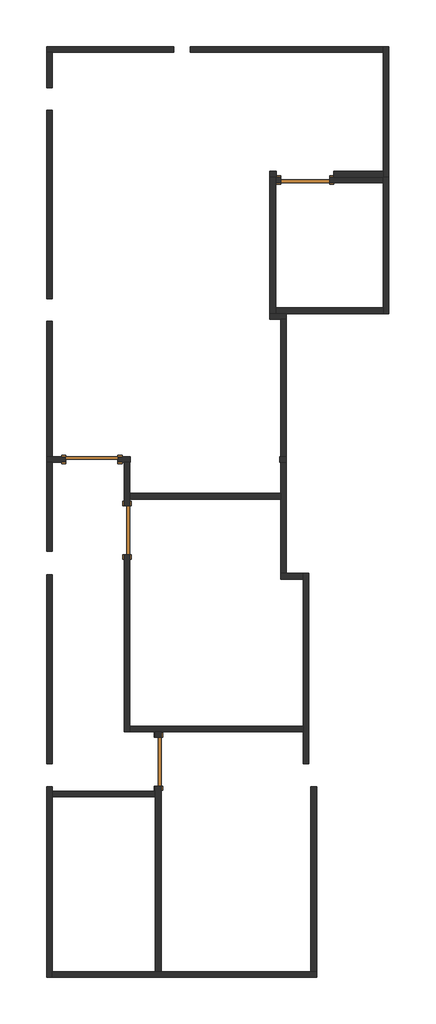
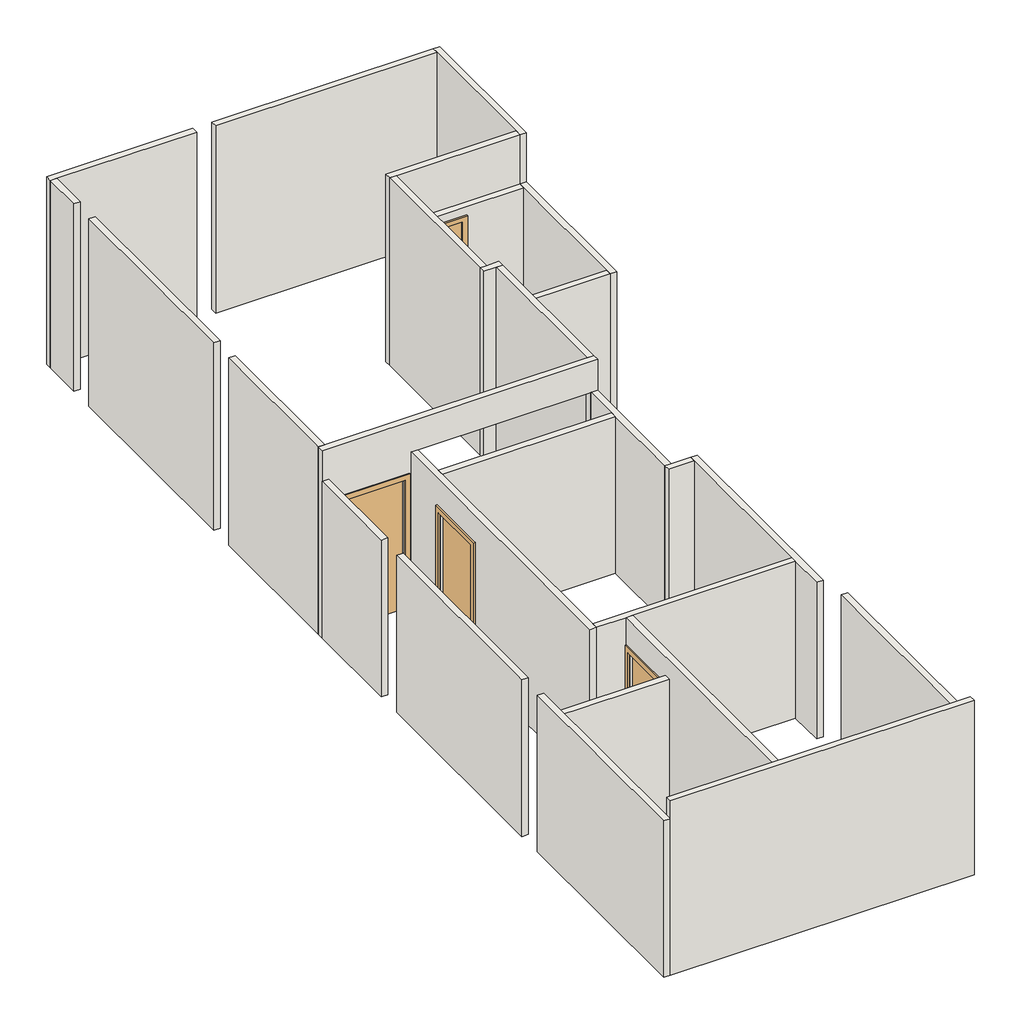
# One storey: 27 walls, 4 doors.
"""IFC4 building model written with IfcOpenShell, lengths in millimetres."""

import ifcopenshell
import ifcopenshell.guid

model = None  # the IFC model being written
_history = None  # IfcOwnerHistory: only IFC2X3 demands one
_inside = {}  # id of a spatial element -> (the spatial element, [elements in it])
_under = {}  # id of a project, library or spatial element -> (it, [spatial elements below it])
_declared = {}  # id of a project -> (the project, [libraries it declares])
_typed = {}  # id of a type object -> (the type object, [elements of that type])
_made_of = {}  # id of a material, layer set ... -> (it, [elements and type objects made of it])


def new_model(schema):
    """Start an empty IFC model of exactly this schema.

    Asked for "IFC4X3", IfcOpenShell would pick the latest addendum, in which some entities
    have other attributes; the version numbers below select the first issue.
    IFC2X3 requires an IfcOwnerHistory on every rooted entity: one is made here for all.
    """
    global model, _history
    if schema == "IFC4X3":
        model = ifcopenshell.file(schema_version=(4, 3, 0, 0))
    else:
        model = ifcopenshell.file(schema=schema)
    _inside.clear()
    _under.clear()
    _declared.clear()
    _typed.clear()
    _made_of.clear()
    _history = None
    if model.schema == "IFC2X3":
        org = make("IfcOrganization", Name="unknown")
        user = make(
            "IfcPersonAndOrganization",
            ThePerson=make("IfcPerson", FamilyName="unknown"),
            TheOrganization=org,
        )
        app = make(
            "IfcApplication",
            ApplicationDeveloper=org,
            Version="unknown",
            ApplicationFullName="unknown",
            ApplicationIdentifier="unknown",
        )
        _history = make(
            "IfcOwnerHistory",
            OwningUser=user,
            OwningApplication=app,
            ChangeAction="ADDED",
            CreationDate=0,
        )
    return model


def make(cls, **values):
    """One entity of the class cls with the attributes given. An attribute that is None is left unset."""
    return model.create_entity(
        cls, **{name: value for name, value in values.items() if value is not None}
    )


def rooted(cls, **values):
    """An entity with a GlobalId (a new one), such as an element, a storey or a relation."""
    return make(cls, GlobalId=ifcopenshell.guid.new(), OwnerHistory=_history, **values)


def si_unit(unit_type, name, prefix=None):
    """IfcSIUnit, for example si_unit("LENGTHUNIT", "METRE", prefix="MILLI")."""
    return make("IfcSIUnit", UnitType=unit_type, Prefix=prefix, Name=name)


def assignment(units):
    """IfcUnitAssignment: the units of a project."""
    return None if units is None else make("IfcUnitAssignment", Units=units)


def point(xyz):
    """IfcCartesianPoint."""
    return None if xyz is None else make("IfcCartesianPoint", Coordinates=xyz)


def direction(xyz):
    """IfcDirection."""
    return None if xyz is None else make("IfcDirection", DirectionRatios=xyz)


def frame(location, z_axis=None, x_axis=None):
    """IfcAxis2Placement3D, a coordinate frame: its origin and axes. An axis left out is left unset."""
    return make(
        "IfcAxis2Placement3D",
        Location=point(location),
        Axis=direction(z_axis),
        RefDirection=direction(x_axis),
    )


def origin():
    """The frame at (0, 0, 0) with its axes left unset."""
    return frame((0.0, 0.0, 0.0))


def origin_with_axes():
    """The frame at (0, 0, 0) with the z axis (0, 0, 1) and the x axis (1, 0, 0) written out."""
    return frame((0.0, 0.0, 0.0), z_axis=(0.0, 0.0, 1.0), x_axis=(1.0, 0.0, 0.0))


def place(relative_to, where):
    """IfcLocalPlacement: puts the frame where relative to a parent placement (None: the world)."""
    return make(
        "IfcLocalPlacement", PlacementRelTo=relative_to, RelativePlacement=where
    )


def context(
    kind, dimensions, precision=None, world=None, true_north=None, identifier=None
):
    """IfcGeometricRepresentationContext, for example the 3D "Model" context."""
    return make(
        "IfcGeometricRepresentationContext",
        ContextIdentifier=identifier,
        ContextType=kind,
        CoordinateSpaceDimension=dimensions,
        Precision=precision,
        WorldCoordinateSystem=world,
        TrueNorth=true_north,
    )


def project(units=None, contexts=None):
    """IfcProject with its units and contexts."""
    return rooted(
        "IfcProject",
        Name="project",
        RepresentationContexts=contexts,
        UnitsInContext=assignment(units),
    )


def spatial(cls, under=None, at=None, **own):
    """A site, building, storey or space (cls), placed at a placement, below another one or the project."""
    s = rooted(cls, ObjectPlacement=at, **own)
    if under is not None:
        _under.setdefault(under.id(), (under, []))[1].append(s)
    return s


def polyline(points):
    """IfcPolyline through the points."""
    return make("IfcPolyline", Points=[point(p) for p in points])


def outline(outer, holes=None, kind="AREA"):
    """IfcArbitraryClosedProfileDef: a profile drawn as a closed curve; with holes, ...WithVoids."""
    if holes is None:
        return make("IfcArbitraryClosedProfileDef", ProfileType=kind, OuterCurve=outer)
    return make(
        "IfcArbitraryProfileDefWithVoids",
        ProfileType=kind,
        OuterCurve=outer,
        InnerCurves=holes,
    )


def extrude(swept, where, along, depth):
    """IfcExtrudedAreaSolid: the profile swept, set in the frame where, extruded along a direction by depth."""
    return make(
        "IfcExtrudedAreaSolid",
        SweptArea=swept,
        Position=where,
        ExtrudedDirection=direction(along),
        Depth=depth,
    )


def faces_of(points, faces, orient=None, outer=None):
    """IfcFace entities. A face is a list of loops; a loop is a list of indices into points, from 0.

    orient and outer hold one flag for each loop. By default every Orientation is true, the
    first loop of a face is its IfcFaceOuterBound and the others are IfcFaceBound.
    """
    made = []
    for i, loops in enumerate(faces):
        bounds = []
        for j, loop in enumerate(loops):
            is_outer = j == 0 if outer is None else outer[i][j]
            bounds.append(
                make(
                    "IfcFaceOuterBound" if is_outer else "IfcFaceBound",
                    Bound=make("IfcPolyLoop", Polygon=[points[k] for k in loop]),
                    Orientation=True if orient is None else orient[i][j],
                )
            )
        made.append(make("IfcFace", Bounds=bounds))
    return made


def faceted_brep(points, faces, orient=None, outer=None, voids=None):
    """IfcFacetedBrep: a solid bounded by flat faces; with voids (closed shells), ...WithVoids."""
    shared = [point(p) for p in points]
    hull = make("IfcClosedShell", CfsFaces=faces_of(shared, faces, orient, outer))
    if voids is None:
        return make("IfcFacetedBrep", Outer=hull)
    return make(
        "IfcFacetedBrepWithVoids",
        Outer=hull,
        Voids=[
            make(cls, CfsFaces=faces_of(shared, fs, o, b)) for cls, fs, o, b in voids
        ],
    )


def shape(context_of_items, identifier, shape_type, items):
    """IfcShapeRepresentation: the items that make up one representation, for example the "Body"."""
    return make(
        "IfcShapeRepresentation",
        ContextOfItems=context_of_items,
        RepresentationIdentifier=identifier,
        RepresentationType=shape_type,
        Items=items,
    )


def source(mapping_origin, context_of_items, identifier, shape_type, items):
    """IfcRepresentationMap: a shape defined once, which mapped items show again and again."""
    return make(
        "IfcRepresentationMap",
        MappingOrigin=mapping_origin,
        MappedRepresentation=shape(context_of_items, identifier, shape_type, items),
    )


def transform(
    local_origin,
    x_axis=None,
    y_axis=None,
    z_axis=None,
    scale=None,
    scale2=None,
    scale3=None,
    uniform=True,
):
    """IfcCartesianTransformationOperator3D, or its non-uniform kind. x_axis, y_axis, z_axis: its Axis1, 2, 3."""
    if uniform:
        return make(
            "IfcCartesianTransformationOperator3D",
            Axis1=direction(x_axis),
            Axis2=direction(y_axis),
            LocalOrigin=point(local_origin),
            Scale=scale,
            Axis3=direction(z_axis),
        )
    return make(
        "IfcCartesianTransformationOperator3DnonUniform",
        Axis1=direction(x_axis),
        Axis2=direction(y_axis),
        LocalOrigin=point(local_origin),
        Scale=scale,
        Axis3=direction(z_axis),
        Scale2=scale2,
        Scale3=scale3,
    )


def mapped(mapping_source, mapping_target):
    """IfcMappedItem: shows the shape of a source again, moved by a transform."""
    return make(
        "IfcMappedItem", MappingSource=mapping_source, MappingTarget=mapping_target
    )


def made_of(thing, what):
    """Note that an element or type object is made of a material, layer set ...; save() writes the relation."""
    if what is not None:
        _made_of.setdefault(what.id(), (what, []))[1].append(thing)
    return thing


def element(
    cls,
    number,
    at=None,
    inside=None,
    cuts=None,
    type_object=None,
    material=None,
    context=None,
    identifier="Body",
    shape_type=None,
    held_by="IfcProductDefinitionShape",
    body=None,
    shapes=None,
    **own,
):
    """One element of the class cls, such as IfcWall. Its Tag is "e" and its number.

    at: its placement. inside: the storey or other place that contains it. cuts: it is an
    opening in that element (IfcRelVoidsElement). A single representation is given by context,
    identifier, shape_type and body (its items); several are given by shapes. held_by: the class
    of the entity that holds the representations. save() writes the other relations.
    """
    e = rooted(cls, Tag="e%d" % number, ObjectPlacement=at, **own)
    if body is not None:
        shapes = [shape(context, identifier, shape_type, body)]
    if shapes is not None:
        e.Representation = make(held_by, Representations=shapes)
    if inside is not None:
        _inside.setdefault(inside.id(), (inside, []))[1].append(e)
    if cuts is not None:
        rooted(
            "IfcRelVoidsElement", RelatingBuildingElement=cuts, RelatedOpeningElement=e
        )
    if type_object is not None:
        _typed.setdefault(type_object.id(), (type_object, []))[1].append(e)
    return made_of(e, material)


def aggregate(whole, parts):
    """IfcRelAggregates: a whole, such as a stair, and the parts it consists of."""
    return rooted("IfcRelAggregates", RelatingObject=whole, RelatedObjects=parts)


def save(model, path):
    """Write the relations noted so far, then the file.

    IfcRelAggregates (storeys below a building ...), IfcRelContainedInSpatialStructure (elements
    in a storey), IfcRelDefinesByType, IfcRelAssociatesMaterial and IfcRelDeclares: one each for
    every whole, place, type object, material and project.
    """
    for whole, parts in _under.values():
        aggregate(whole, parts)
    for where, things in _inside.values():
        rooted(
            "IfcRelContainedInSpatialStructure",
            RelatedElements=things,
            RelatingStructure=where,
        )
    for kind, things in _typed.values():
        rooted("IfcRelDefinesByType", RelatedObjects=things, RelatingType=kind)
    for what, things in _made_of.values():
        rooted("IfcRelAssociatesMaterial", RelatedObjects=things, RelatingMaterial=what)
    for by, libraries in _declared.values():
        rooted("IfcRelDeclares", RelatingContext=by, RelatedDefinitions=libraries)
    model.write(path)


def m_single_flush_0864_x_2032mm_0d7903e5(model_context):
    return source(origin(), model_context, "Body", "SweptSolid", [
        extrude(outline(polyline([(2108.0, -508.0), (0.0, -508.0), (0.0, -432.0), (2032.0, -432.0), (2032.0, 432.0), (0.0, 432.0), (0.0, 508.0), (2108.0, 508.0), (2108.0, -508.0)])), frame((0.0, -75.0, 0.0), z_axis=(0.0, 1.0, 0.0), x_axis=(0.0, 0.0, 1.0)), (0.0, 0.0, 1.0), 25.0),
        extrude(outline(polyline([(2108.0, 508.0), (2108.0, -508.0), (0.0, -508.0), (0.0, -432.0), (2032.0, -432.0), (2032.0, 432.0), (0.0, 432.0), (0.0, 508.0), (2108.0, 508.0)])), frame((0.0, 50.0, 0.0), z_axis=(0.0, 1.0, 0.0), x_axis=(0.0, 0.0, 1.0)), (0.0, 0.0, 1.0), 25.0),
        extrude(outline(polyline([(432.0, 1.0), (432.0, -50.0), (-432.0, -50.0), (-432.0, 1.0), (432.0, 1.0)])), origin_with_axes(), (0.0, 0.0, 1.0), 2032.0),
    ])


def m_single_flush_0864_x_2032mm_252f296b(model_context):
    return source(origin(), model_context, "Body", "SweptSolid", [
        extrude(outline(polyline([(2108.0, -508.0), (0.0, -508.0), (0.0, -432.0), (2032.0, -432.0), (2032.0, 432.0), (0.0, 432.0), (0.0, 508.0), (2108.0, 508.0), (2108.0, -508.0)])), frame((0.0, 50.0, 0.0), z_axis=(0.0, 1.0, 0.0), x_axis=(0.0, 0.0, 1.0)), (0.0, 0.0, 1.0), 25.0),
        extrude(outline(polyline([(2108.0, 508.0), (2108.0, -508.0), (0.0, -508.0), (0.0, -432.0), (2032.0, -432.0), (2032.0, 432.0), (0.0, 432.0), (0.0, 508.0), (2108.0, 508.0)])), frame((0.0, -75.0, 0.0), z_axis=(0.0, 1.0, 0.0), x_axis=(0.0, 0.0, 1.0)), (0.0, 0.0, 1.0), 25.0),
        extrude(outline(polyline([(432.0, -1.0), (-432.0, -1.0), (-432.0, 50.0), (432.0, 50.0), (432.0, -1.0)])), origin_with_axes(), (0.0, 0.0, 1.0), 2032.0),
    ])


def m_single_flush_0915_x_2134mm_17617764(model_context):
    return source(origin(), model_context, "Body", "SweptSolid", [
        extrude(outline(polyline([(2210.0, -533.5), (0.0, -533.5), (0.0, -457.5), (2134.0, -457.5), (2134.0, 457.5), (0.0, 457.5), (0.0, 533.5), (2210.0, 533.5), (2210.0, -533.5)])), frame((0.0, -75.0, 0.0), z_axis=(0.0, 1.0, 0.0), x_axis=(0.0, 0.0, 1.0)), (0.0, 0.0, 1.0), 25.0),
        extrude(outline(polyline([(2210.0, 533.5), (2210.0, -533.5), (0.0, -533.5), (0.0, -457.5), (2134.0, -457.5), (2134.0, 457.5), (0.0, 457.5), (0.0, 533.5), (2210.0, 533.5)])), frame((0.0, 50.0, 0.0), z_axis=(0.0, 1.0, 0.0), x_axis=(0.0, 0.0, 1.0)), (0.0, 0.0, 1.0), 25.0),
        extrude(outline(polyline([(457.5, 1.0), (457.5, -50.0), (-457.5, -50.0), (-457.5, 1.0), (457.5, 1.0)])), origin_with_axes(), (0.0, 0.0, 1.0), 2134.0),
    ])


model = new_model("IFC4")

# Units and contexts
model_context = context("Model", 3, world=origin())
ifc_project = project(units=[si_unit("LENGTHUNIT", "METRE", prefix="MILLI")], contexts=[model_context])

# Site, building, storey
site = spatial("IfcSite", under=ifc_project)
building = spatial("IfcBuilding", under=site)
storey = spatial("IfcBuildingStorey", under=building, Name="Suelo de apartemento", Elevation=250.0)

# Doors
placement = place(None, origin())
m_single_flush_0864_x_2032mm_shape = m_single_flush_0864_x_2032mm_0d7903e5(model_context)
element("IfcDoor", 1, ObjectType="M_Single-Flush : 0864 x 2032mm", at=placement, inside=storey, context=model_context, shape_type="MappedRepresentation", body=[
    mapped(m_single_flush_0864_x_2032mm_shape, transform((7037.3508412, 6265.939444, 250.0), x_axis=(0.0, 1.0, 0.0), y_axis=(-1.0, 0.0, 0.0), z_axis=(0.0, 0.0, 1.0))),
])
element("IfcDoor", 2, ObjectType="M_Single-Flush : 0864 x 2032mm", at=placement, inside=storey, context=model_context, shape_type="MappedRepresentation", body=[
    mapped(m_single_flush_0864_x_2032mm_shape, transform((7592.3508412, 2190.939444, 250.0), x_axis=(0.0, 1.0, 0.0), y_axis=(-1.0, 0.0, 0.0), z_axis=(0.0, 0.0, 1.0))),
])
m_single_flush_0864_x_2032mm_2_shape = m_single_flush_0864_x_2032mm_252f296b(model_context)
element("IfcDoor", 3, ObjectType="M_Single-Flush : 0864 x 2032mm", at=placement, inside=storey, context=model_context, shape_type="MappedRepresentation", body=[
    mapped(m_single_flush_0864_x_2032mm_2_shape, transform((10177.3508412, 12440.939444, 250.0), x_axis=(-1.0, 0.0, 0.0), y_axis=(0.0, -1.0, 0.0), z_axis=(0.0, 0.0, 1.0))),
])
m_single_flush_0915_x_2134mm_shape = m_single_flush_0915_x_2134mm_17617764(model_context)
element("IfcDoor", 4, ObjectType="M_Single-Flush : 0915 x 2134mm", at=placement, inside=storey, context=model_context, shape_type="MappedRepresentation", body=[
    mapped(m_single_flush_0915_x_2134mm_shape, transform((6422.3508412, 7515.939444, 250.0), x_axis=(-1.0, 0.0, 0.0), y_axis=(0.0, -1.0, 0.0), z_axis=(0.0, 0.0, 1.0))),
])

# Walls
element("IfcWall", 5, ObjectType="Steel Frame 100mm", at=placement, inside=storey, context=model_context, shape_type="Brep", body=[
    faceted_brep([(5722.3508412, -1614.060556, 250.0), (5722.3508412, -1514.060556, 250.0), (5722.3508412, 1565.939444, 250.0), (5722.3508412, 1665.939444, 250.0), (5722.3508412, 1745.939444, 250.0), (5722.3508412, 1745.939444, 2790.0), (5722.3508412, -1614.060556, 2790.0), (5622.3508412, -1614.060556, 250.0), (5622.3508412, -1614.060556, 2790.0), (5622.3508412, 1745.939444, 2790.0), (5622.3508412, 1745.939444, 250.0)], [[[0, 1, 2, 3, 4, 5, 6]], [[7, 8, 9, 10]], [[4, 3, 2, 1, 0, 7, 10]], [[5, 4, 10, 9]], [[6, 5, 9, 8]], [[0, 6, 8, 7]]]),
])
element("IfcWall", 6, ObjectType="Steel Frame 100mm", at=placement, inside=storey, context=model_context, shape_type="SweptSolid", body=[
    extrude(outline(polyline([(5722.3508412, 5485.939444), (5722.3508412, 2155.939444), (5622.3508412, 2155.939444), (5622.3508412, 5485.939444), (5722.3508412, 5485.939444)])), frame((0.0, 0.0, 250.0), z_axis=(0.0, 0.0, 1.0), x_axis=(1.0, 0.0, 0.0)), (0.0, 0.0, 1.0), 2540.0),
])
element("IfcWall", 7, ObjectType="Steel Frame 100mm", at=placement, inside=storey, context=model_context, shape_type="SweptSolid", body=[
    extrude(outline(polyline([(5722.3508412, 9945.939444), (5722.3508412, 7565.939444), (5622.3508412, 7565.939444), (5622.3508412, 9945.939444), (5722.3508412, 9945.939444)])), frame((0.0, 0.0, 250.0), z_axis=(0.0, 0.0, 1.0), x_axis=(1.0, 0.0, 0.0)), (0.0, 0.0, 1.0), 3040.0),
])
element("IfcWall", 8, ObjectType="Steel Frame 100mm", at=placement, inside=storey, context=model_context, shape_type="SweptSolid", body=[
    extrude(outline(polyline([(5722.3508412, 13665.939444), (5722.3508412, 10345.939444), (5622.3508412, 10345.939444), (5622.3508412, 13665.939444), (5722.3508412, 13665.939444)])), frame((0.0, 0.0, 250.0), z_axis=(0.0, 0.0, 1.0), x_axis=(1.0, 0.0, 0.0)), (0.0, 0.0, 1.0), 3040.0),
])
element("IfcWall", 9, ObjectType="Steel Frame 100mm", at=placement, inside=storey, context=model_context, shape_type="SweptSolid", body=[
    extrude(outline(polyline([(5722.3508412, 14690.939444), (5722.3508412, 14065.939444), (5622.3508412, 14065.939444), (5622.3508412, 14690.939444), (5722.3508412, 14690.939444)])), frame((0.0, 0.0, 250.0), z_axis=(0.0, 0.0, 1.0), x_axis=(1.0, 0.0, 0.0)), (0.0, 0.0, 1.0), 3040.0),
])
element("IfcWall", 10, ObjectType="Steel Frame 100mm", at=placement, inside=storey, context=model_context, shape_type="Brep", body=[
    faceted_brep([(5622.3508412, 14690.939444, 250.0), (5722.3508412, 14690.939444, 250.0), (7867.3508412, 14690.939444, 250.0), (7867.3508412, 14690.939444, 3290.0), (5722.3508412, 14690.939444, 3290.0), (5622.3508412, 14690.939444, 3290.0), (5622.3508412, 14790.939444, 250.0), (5622.3508412, 14790.939444, 3290.0), (7867.3508412, 14790.939444, 3290.0), (7867.3508412, 14790.939444, 250.0)], [[[0, 1, 2, 3, 4, 5]], [[6, 7, 8, 9]], [[2, 1, 0, 6, 9]], [[3, 2, 9, 8]], [[5, 4, 3, 8, 7]], [[0, 5, 7, 6]]]),
])
element("IfcWall", 11, ObjectType="Steel Frame 100mm", at=placement, inside=storey, context=model_context, shape_type="Brep", body=[
    faceted_brep([(11657.3508412, 12490.939444, 3290.0), (11657.3508412, 12490.939444, 2490.0), (11657.3508412, 12490.939444, 250.0), (11657.3508412, 14790.939444, 250.0), (11657.3508412, 14790.939444, 3290.0), (11557.3508412, 12490.939444, 250.0), (11557.3508412, 12490.939444, 2490.0), (11557.3508412, 12490.939444, 3290.0), (11557.3508412, 12590.939444, 3290.0), (11557.3508412, 14690.939444, 3290.0), (11557.3508412, 14790.939444, 3290.0), (11557.3508412, 14790.939444, 250.0), (11557.3508412, 14690.939444, 250.0), (11557.3508412, 12590.939444, 250.0)], [[[0, 1, 2, 3, 4]], [[5, 6, 7, 8, 9, 10, 11, 12, 13]], [[3, 2, 5, 13, 12, 11]], [[0, 4, 10, 9, 8, 7]], [[4, 3, 11, 10]], [[0, 7, 6, 5, 2, 1]]]),
])
element("IfcWall", 12, ObjectType="Steel Frame 100mm", at=placement, inside=storey, context=model_context, shape_type="SweptSolid", body=[
    extrude(outline(polyline([(11557.3508412, 14690.939444), (8157.3508412, 14690.939444), (8157.3508412, 14790.939444), (11557.3508412, 14790.939444), (11557.3508412, 14690.939444)])), frame((0.0, 0.0, 250.0), z_axis=(0.0, 0.0, 1.0), x_axis=(1.0, 0.0, 0.0)), (0.0, 0.0, 1.0), 3040.0),
])
element("IfcWall", 13, ObjectType="Steel Frame 100mm", at=placement, inside=storey, context=model_context, shape_type="Brep", body=[
    faceted_brep([(9557.3508412, 12590.939444, 250.0), (9557.3508412, 12590.939444, 3290.0), (11557.3508412, 12590.939444, 3290.0), (11557.3508412, 12590.939444, 250.0), (10687.3508412, 12590.939444, 250.0), (10687.3508412, 12590.939444, 2360.0), (9667.3508412, 12590.939444, 2360.0), (9667.3508412, 12590.939444, 250.0), (9557.3508412, 12490.939444, 3290.0), (9557.3508412, 12490.939444, 250.0), (9657.3508412, 12490.939444, 250.0), (9667.3508412, 12490.939444, 250.0), (9667.3508412, 12490.939444, 2360.0), (10687.3508412, 12490.939444, 2360.0), (10687.3508412, 12490.939444, 250.0), (11557.3508412, 12490.939444, 250.0), (11557.3508412, 12490.939444, 3290.0), (9657.3508412, 12490.939444, 3290.0)], [[[0, 1, 2, 3, 4, 5, 6, 7]], [[8, 9, 10, 11, 12, 13, 14, 15, 16, 17]], [[3, 15, 14, 4]], [[9, 0, 7, 11, 10]], [[2, 1, 8, 17, 16]], [[1, 0, 9, 8]], [[2, 16, 15, 3]], [[5, 13, 12, 6]], [[13, 5, 4, 14]], [[6, 12, 11, 7]]]),
])
element("IfcWall", 14, ObjectType="Steel Frame 100mm", at=placement, inside=storey, context=model_context, shape_type="Brep", body=[
    faceted_brep([(9557.3508412, 12490.939444, 250.0), (9557.3508412, 10085.939444, 250.0), (9557.3508412, 10085.939444, 3290.0), (9557.3508412, 12490.939444, 3290.0), (9657.3508412, 12490.939444, 250.0), (9657.3508412, 12490.939444, 2490.0), (9657.3508412, 12490.939444, 3290.0), (9657.3508412, 10085.939444, 3290.0), (9657.3508412, 10085.939444, 2490.0), (9657.3508412, 10085.939444, 250.0), (9657.3508412, 10185.939444, 250.0), (9657.3508412, 12390.939444, 250.0)], [[[0, 1, 2, 3]], [[4, 5, 6, 7, 8, 9, 10, 11]], [[1, 0, 4, 11, 10, 9]], [[3, 2, 7, 6]], [[0, 3, 6, 5, 4]], [[2, 1, 9, 8, 7]]]),
])
element("IfcWall", 15, ObjectType="Steel Frame 100mm", at=placement, inside=storey, context=model_context, shape_type="Brep", body=[
    faceted_brep([(9557.3508412, 9985.939444, 250.0), (9747.3508412, 9985.939444, 250.0), (9847.3508412, 9985.939444, 250.0), (9847.3508412, 9985.939444, 3290.0), (9747.3508412, 9985.939444, 3290.0), (9557.3508412, 9985.939444, 3290.0), (9557.3508412, 10085.939444, 250.0), (9557.3508412, 10085.939444, 3290.0), (9657.3508412, 10085.939444, 3290.0), (9847.3508412, 10085.939444, 3290.0), (9847.3508412, 10085.939444, 250.0), (9657.3508412, 10085.939444, 250.0)], [[[0, 1, 2, 3, 4, 5]], [[6, 7, 8, 9, 10, 11]], [[2, 1, 0, 6, 11, 10]], [[5, 4, 3, 9, 8, 7]], [[0, 5, 7, 6]], [[3, 2, 10, 9]]]),
])
element("IfcWall", 16, ObjectType="Steel Frame 100mm", at=placement, inside=storey, context=model_context, shape_type="Brep", body=[
    faceted_brep([(11557.3508412, 12490.939444, 250.0), (11557.3508412, 12390.939444, 250.0), (11557.3508412, 10185.939444, 250.0), (11557.3508412, 10085.939444, 250.0), (11557.3508412, 10085.939444, 2490.0), (11557.3508412, 10185.939444, 2490.0), (11557.3508412, 12390.939444, 2490.0), (11557.3508412, 12490.939444, 2490.0), (11657.3508412, 12490.939444, 250.0), (11657.3508412, 12490.939444, 2490.0), (11657.3508412, 10085.939444, 2490.0), (11657.3508412, 10085.939444, 250.0)], [[[0, 1, 2, 3, 4, 5, 6, 7]], [[8, 9, 10, 11]], [[3, 2, 1, 0, 8, 11]], [[7, 6, 5, 4, 10, 9]], [[0, 7, 9, 8]], [[4, 3, 11, 10]]]),
])
element("IfcWall", 17, ObjectType="Steel Frame 100mm", at=placement, inside=storey, context=model_context, shape_type="SweptSolid", body=[
    extrude(outline(polyline([(9657.3508412, 10185.939444), (11557.3508412, 10185.939444), (11557.3508412, 10085.939444), (9657.3508412, 10085.939444), (9657.3508412, 10185.939444)])), frame((0.0, 0.0, 250.0), z_axis=(0.0, 0.0, 1.0), x_axis=(1.0, 0.0, 0.0)), (0.0, 0.0, 1.0), 2240.0),
])
element("IfcWall", 18, ObjectType="Steel Frame 100mm", at=placement, inside=storey, context=model_context, shape_type="SweptSolid", body=[
    extrude(outline(polyline([(250.0, 9657.3508412), (250.0, 9745.3508412), (2282.0, 9745.3508412), (2282.0, 10609.3508412), (250.0, 10609.3508412), (250.0, 11557.3508412), (2490.0, 11557.3508412), (2490.0, 9657.3508412), (250.0, 9657.3508412)])), frame((0.0, 12390.939444, 0.0), z_axis=(0.0, 1.0, 0.0), x_axis=(0.0, 0.0, 1.0)), (0.0, 0.0, 1.0), 100.0),
])
element("IfcWall", 19, ObjectType="Steel Frame 100mm", at=placement, inside=storey, context=model_context, shape_type="Brep", body=[
    faceted_brep([(9847.3508412, 5505.939444, 250.0), (9847.3508412, 7465.939444, 250.0), (9847.3508412, 7465.939444, 2790.0), (9847.3508412, 5505.939444, 2790.0), (9747.3508412, 5505.939444, 250.0), (9747.3508412, 5505.939444, 2790.0), (9747.3508412, 6815.939444, 2790.0), (9747.3508412, 6915.939444, 2790.0), (9747.3508412, 7465.939444, 2790.0), (9747.3508412, 7465.939444, 250.0), (9747.3508412, 6915.939444, 250.0), (9747.3508412, 6815.939444, 250.0)], [[[0, 1, 2, 3]], [[4, 5, 6, 7, 8, 9, 10, 11]], [[1, 0, 4, 11, 10, 9]], [[3, 2, 8, 7, 6, 5]], [[0, 3, 5, 4]], [[2, 1, 9, 8]]]),
])
element("IfcWall", 20, ObjectType="Steel Frame 100mm", at=placement, inside=storey, context=model_context, shape_type="SweptSolid", body=[
    extrude(outline(polyline([(9847.3508412, 9985.939444), (9847.3508412, 7565.939444), (9747.3508412, 7565.939444), (9747.3508412, 9985.939444), (9847.3508412, 9985.939444)])), frame((0.0, 0.0, 250.0), z_axis=(0.0, 0.0, 1.0), x_axis=(1.0, 0.0, 0.0)), (0.0, 0.0, 1.0), 3040.0),
])
element("IfcWall", 21, ObjectType="Steel Frame 100mm", at=placement, inside=storey, context=model_context, shape_type="Brep", body=[
    faceted_brep([(5964.8508412, 7565.939444, 2384.0), (5964.8508412, 7565.939444, 250.0), (5722.3508412, 7565.939444, 250.0), (5622.3508412, 7565.939444, 250.0), (5622.3508412, 7565.939444, 3290.0), (5722.3508412, 7565.939444, 3290.0), (9747.3508412, 7565.939444, 3290.0), (9847.3508412, 7565.939444, 3290.0), (9847.3508412, 7565.939444, 250.0), (9747.3508412, 7565.939444, 250.0), (9732.3508412, 7565.939444, 250.0), (9732.3508412, 7565.939444, 2790.0), (7095.0342555, 7565.939444, 2790.0), (7095.0342555, 7565.939444, 250.0), (6879.8508412, 7565.939444, 250.0), (6879.8508412, 7565.939444, 2384.0), (5622.3508412, 7465.939444, 250.0), (5722.3508412, 7465.939444, 250.0), (5964.8508412, 7465.939444, 250.0), (5964.8508412, 7465.939444, 2384.0), (6879.8508412, 7465.939444, 2384.0), (6879.8508412, 7465.939444, 250.0), (6987.3508412, 7465.939444, 250.0), (7087.3508412, 7465.939444, 250.0), (7095.0342555, 7465.939444, 250.0), (7095.0342555, 7465.939444, 2790.0), (9732.3508412, 7465.939444, 2790.0), (9732.3508412, 7465.939444, 250.0), (9747.3508412, 7465.939444, 250.0), (9847.3508412, 7465.939444, 250.0), (9847.3508412, 7465.939444, 2790.0), (9847.3508412, 7465.939444, 3290.0), (5622.3508412, 7465.939444, 3290.0), (5622.3508412, 7465.939444, 2790.0)], [[[0, 1, 2, 3, 4, 5, 6, 7, 8, 9, 10, 11, 12, 13, 14, 15]], [[16, 17, 18, 19, 20, 21, 22, 23, 24, 25, 26, 27, 28, 29, 30, 31, 32, 33]], [[8, 29, 28, 27, 10, 9]], [[14, 13, 24, 23, 22, 21]], [[3, 2, 1, 18, 17, 16]], [[7, 6, 5, 4, 32, 31]], [[19, 18, 1, 0]], [[20, 19, 0, 15]], [[21, 20, 15, 14]], [[3, 16, 33, 32, 4]], [[7, 31, 30, 29, 8]], [[11, 26, 25, 12]], [[26, 11, 10, 27]], [[12, 25, 24, 13]]]),
])
element("IfcWall", 22, ObjectType="Steel Frame 100mm", at=placement, inside=storey, context=model_context, shape_type="Brep", body=[
    faceted_brep([(5722.3508412, -1614.060556, 250.0), (10382.3508412, -1614.060556, 250.0), (10382.3508412, -1614.060556, 3080.0), (5722.3508412, -1614.060556, 3080.0), (5722.3508412, -1614.060556, 2790.0), (5722.3508412, -1514.060556, 250.0), (5722.3508412, -1514.060556, 3080.0), (10382.3508412, -1514.060556, 3080.0), (10382.3508412, -1514.060556, 2790.0), (10382.3508412, -1514.060556, 250.0), (10282.3508412, -1514.060556, 250.0), (7642.3508412, -1514.060556, 250.0), (7542.3508412, -1514.060556, 250.0)], [[[0, 1, 2, 3, 4]], [[5, 6, 7, 8, 9, 10, 11, 12]], [[1, 0, 5, 12, 11, 10, 9]], [[3, 2, 7, 6]], [[0, 4, 3, 6, 5]], [[2, 1, 9, 8, 7]]]),
])
element("IfcWall", 23, ObjectType="Steel Frame 100mm", at=placement, inside=storey, context=model_context, shape_type="SweptSolid", body=[
    extrude(outline(polyline([(10382.3508412, 1745.939444), (10382.3508412, -1514.060556), (10282.3508412, -1514.060556), (10282.3508412, 1745.939444), (10382.3508412, 1745.939444)])), frame((0.0, 0.0, 250.0), z_axis=(0.0, 0.0, 1.0), x_axis=(1.0, 0.0, 0.0)), (0.0, 0.0, 1.0), 2540.0),
])
element("IfcWall", 24, ObjectType="Steel Frame 100mm", at=placement, inside=storey, context=model_context, shape_type="Brep", body=[
    faceted_brep([(7642.3508412, 2622.939444, 2282.0), (7642.3508412, 2622.939444, 250.0), (7642.3508412, 2715.939444, 250.0), (7642.3508412, 2715.939444, 2790.0), (7642.3508412, -1514.060556, 2790.0), (7642.3508412, -1514.060556, 250.0), (7642.3508412, 1758.939444, 250.0), (7642.3508412, 1758.939444, 2282.0), (7542.3508412, 2715.939444, 250.0), (7542.3508412, 2622.939444, 250.0), (7542.3508412, 2622.939444, 2282.0), (7542.3508412, 1758.939444, 2282.0), (7542.3508412, 1758.939444, 250.0), (7542.3508412, 1665.939444, 250.0), (7542.3508412, 1565.939444, 250.0), (7542.3508412, -1514.060556, 250.0), (7542.3508412, -1514.060556, 2790.0), (7542.3508412, 2715.939444, 2790.0)], [[[0, 1, 2, 3, 4, 5, 6, 7]], [[8, 9, 10, 11, 12, 13, 14, 15, 16, 17]], [[6, 5, 15, 14, 13, 12]], [[2, 1, 9, 8]], [[4, 3, 17, 16]], [[5, 4, 16, 15]], [[3, 2, 8, 17]], [[10, 9, 1, 0]], [[11, 10, 0, 7]], [[12, 11, 7, 6]]]),
])
element("IfcWall", 25, ObjectType="Steel Frame 100mm", at=placement, inside=storey, context=model_context, shape_type="Brep", body=[
    faceted_brep([(7087.3508412, 6697.939444, 2282.0), (7087.3508412, 6697.939444, 250.0), (7087.3508412, 6815.939444, 250.0), (7087.3508412, 6915.939444, 250.0), (7087.3508412, 7465.939444, 250.0), (7087.3508412, 7465.939444, 2790.0), (7087.3508412, 6915.939444, 2790.0), (7087.3508412, 6815.939444, 2790.0), (7087.3508412, 2815.939444, 2790.0), (7087.3508412, 2715.939444, 2790.0), (7087.3508412, 2715.939444, 250.0), (7087.3508412, 2815.939444, 250.0), (7087.3508412, 5833.939444, 250.0), (7087.3508412, 5833.939444, 2282.0), (6987.3508412, 7465.939444, 250.0), (6987.3508412, 6697.939444, 250.0), (6987.3508412, 6697.939444, 2282.0), (6987.3508412, 5833.939444, 2282.0), (6987.3508412, 5833.939444, 250.0), (6987.3508412, 2715.939444, 250.0), (6987.3508412, 2715.939444, 2790.0), (6987.3508412, 7465.939444, 2790.0)], [[[0, 1, 2, 3, 4, 5, 6, 7, 8, 9, 10, 11, 12, 13]], [[14, 15, 16, 17, 18, 19, 20, 21]], [[12, 11, 10, 19, 18]], [[4, 3, 2, 1, 15, 14]], [[9, 8, 7, 6, 5, 21, 20]], [[5, 4, 14, 21]], [[10, 9, 20, 19]], [[16, 15, 1, 0]], [[17, 16, 0, 13]], [[18, 17, 13, 12]]]),
])
element("IfcWall", 26, ObjectType="Steel Frame 100mm", at=placement, inside=storey, context=model_context, shape_type="Brep", body=[
    faceted_brep([(10242.3508412, 2155.939444, 250.0), (10242.3508412, 5505.939444, 250.0), (10242.3508412, 5505.939444, 2790.0), (10242.3508412, 2155.939444, 2790.0), (10142.3508412, 2155.939444, 250.0), (10142.3508412, 2155.939444, 2790.0), (10142.3508412, 2715.939444, 2790.0), (10142.3508412, 2815.939444, 2790.0), (10142.3508412, 5405.939444, 2790.0), (10142.3508412, 5505.939444, 2790.0), (10142.3508412, 5505.939444, 250.0), (10142.3508412, 5405.939444, 250.0), (10142.3508412, 2815.939444, 250.0), (10142.3508412, 2715.939444, 250.0)], [[[0, 1, 2, 3]], [[4, 5, 6, 7, 8, 9, 10, 11, 12, 13]], [[1, 0, 4, 13, 12, 11, 10]], [[3, 2, 9, 8, 7, 6, 5]], [[0, 3, 5, 4]], [[2, 1, 10, 9]]]),
])
element("IfcWall", 27, ObjectType="Steel Frame 100mm", at=placement, inside=storey, context=model_context, shape_type="Brep", body=[
    faceted_brep([(10142.3508412, 5505.939444, 250.0), (9847.3508412, 5505.939444, 250.0), (9747.3508412, 5505.939444, 250.0), (9747.3508412, 5505.939444, 2790.0), (9847.3508412, 5505.939444, 2790.0), (10142.3508412, 5505.939444, 2790.0), (10142.3508412, 5405.939444, 250.0), (10142.3508412, 5405.939444, 2790.0), (9747.3508412, 5405.939444, 2790.0), (9747.3508412, 5405.939444, 250.0)], [[[0, 1, 2, 3, 4, 5]], [[6, 7, 8, 9]], [[2, 1, 0, 6, 9]], [[5, 4, 3, 8, 7]], [[0, 5, 7, 6]], [[3, 2, 9, 8]]]),
])
element("IfcWall", 28, ObjectType="Steel Frame 100mm", at=placement, inside=storey, context=model_context, shape_type="Brep", body=[
    faceted_brep([(7087.3508412, 2715.939444, 250.0), (7542.3508412, 2715.939444, 250.0), (7642.3508412, 2715.939444, 250.0), (10142.3508412, 2715.939444, 250.0), (10142.3508412, 2715.939444, 2790.0), (7642.3508412, 2715.939444, 2790.0), (7542.3508412, 2715.939444, 2790.0), (7087.3508412, 2715.939444, 2790.0), (7087.3508412, 2815.939444, 250.0), (7087.3508412, 2815.939444, 2790.0), (10142.3508412, 2815.939444, 2790.0), (10142.3508412, 2815.939444, 250.0)], [[[0, 1, 2, 3, 4, 5, 6, 7]], [[8, 9, 10, 11]], [[3, 2, 1, 0, 8, 11]], [[7, 6, 5, 4, 10, 9]], [[0, 7, 9, 8]], [[4, 3, 11, 10]]]),
])
element("IfcWall", 29, ObjectType="Steel Frame 100mm", at=placement, inside=storey, context=model_context, shape_type="SweptSolid", body=[
    extrude(outline(polyline([(9747.3508412, 6815.939444), (7087.3508412, 6815.939444), (7087.3508412, 6915.939444), (9747.3508412, 6915.939444), (9747.3508412, 6815.939444)])), frame((0.0, 0.0, 250.0), z_axis=(0.0, 0.0, 1.0), x_axis=(1.0, 0.0, 0.0)), (0.0, 0.0, 1.0), 2540.0),
])
element("IfcWall", 30, ObjectType="Steel Frame 100mm", at=placement, inside=storey, context=model_context, shape_type="SweptSolid", body=[
    extrude(outline(polyline([(5722.3508412, 1665.939444), (7542.3508412, 1665.939444), (7542.3508412, 1565.939444), (5722.3508412, 1565.939444), (5722.3508412, 1665.939444)])), frame((0.0, 0.0, 250.0), z_axis=(0.0, 0.0, 1.0), x_axis=(1.0, 0.0, 0.0)), (0.0, 0.0, 1.0), 2240.0),
])
element("IfcWall", 31, ObjectType="Steel Frame 100mm", at=placement, inside=storey, context=model_context, shape_type="SweptSolid", body=[
    extrude(outline(polyline([(5722.3508412, 7465.939444), (5722.3508412, 5895.939444), (5622.3508412, 5895.939444), (5622.3508412, 7465.939444), (5722.3508412, 7465.939444)])), frame((0.0, 0.0, 250.0), z_axis=(0.0, 0.0, 1.0), x_axis=(1.0, 0.0, 0.0)), (0.0, 0.0, 1.0), 2540.0),
])

save(model, "model.ifc")

# Revit data of these elements
# Type "M_Single-Flush : 0864 x 2032mm"
#   Type Mark = "21"
#   Thickness = 5.1 cm
#   Height = 203.2 cm
#   Trim Projection Ext = 2.5 cm
#   Trim Projection Int = 2.5 cm
#   Trim Width = 7.6 cm
#   Width = 86.4 cm
#   Door Material = Door - Panel
#   Frame Material = Door - Frame
#   Function = (empty or 0)
#   Wall Closure = (empty or 0)
# Type "M_Single-Flush : 0915 x 2134mm"
#   Type Mark = "15"
#   Thickness = 5.1 cm
#   Height = 213.4 cm
#   Trim Projection Ext = 2.5 cm
#   Trim Projection Int = 2.5 cm
#   Trim Width = 7.6 cm
#   Width = 91.5 cm
#   Door Material = Door - Panel
#   Frame Material = Door - Frame
#   Function = (empty or 0)
#   Wall Closure = (empty or 0)
# Type "Steel Frame 100mm"
#   Layers, outside or top first: 10 cm no material (function 1)
# Elements 1, 2, 3 (IfcDoor, "M_Single-Flush : 0864 x 2032mm")
#   Phase Created = New Construction
#   Materials on its faces: "Door - Frame", "Door - Panel"
# Element 4 (IfcDoor, "M_Single-Flush : 0915 x 2134mm")
#   Phase Created = New Construction
#   Materials on its faces: "Door - Frame", "Door - Panel"
# Elements 5, 6, 19, 23, 24, 25, 26, 27, 28, 29, 31 (IfcWall, "Steel Frame 100mm")
#   Top Offset = 0 cm
#   Base Offset = 0 cm
#   wall height = 254 cm
#   Phase Created = New Construction
#   Base Constraint = Suelo de apartemento
#   Top Constraint = Techo de dormitorios
#   Materials on its faces: "Default Wall"
# Elements 7, 8, 9, 10, 11, 12, 13, 14, 15, 20, 21 (IfcWall, "Steel Frame 100mm")
#   Top Offset = 0 cm
#   Base Offset = 0 cm
#   wall height = 304 cm
#   Phase Created = New Construction
#   Base Constraint = Suelo de apartemento
#   Top Constraint = Techo de sala
#   Materials on its faces: "Default Wall"
# Elements 16, 17, 18, 30 (IfcWall, "Steel Frame 100mm")
#   Top Offset = 0 cm
#   Base Offset = 0 cm
#   wall height = 224 cm
#   Phase Created = New Construction
#   Base Constraint = Suelo de apartemento
#   Top Constraint = Techo de bano
#   Materials on its faces: "Default Wall"
# Element 22 (IfcWall, "Steel Frame 100mm")
#   Top Offset = 0 cm
#   Base Offset = 0 cm
#   wall height = 283 cm
#   Phase Created = New Construction
#   Base Constraint = Suelo de apartemento
#   Top Constraint = Altura de entrada
#   Materials on its faces: "Default Wall"
# Materials
#   "Door - Panel": class "Wood", colour RGB 114 82 51, transparency 0
#   "Door - Frame": class "Miscellaneous", colour RGB 153 76 43, transparency 0
#   "Default Wall": class "Miscellaneous", colour RGB 80 80 80, transparency 0
